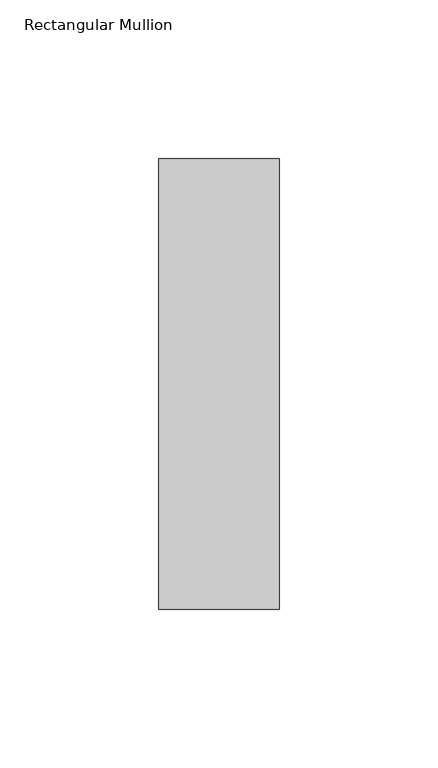
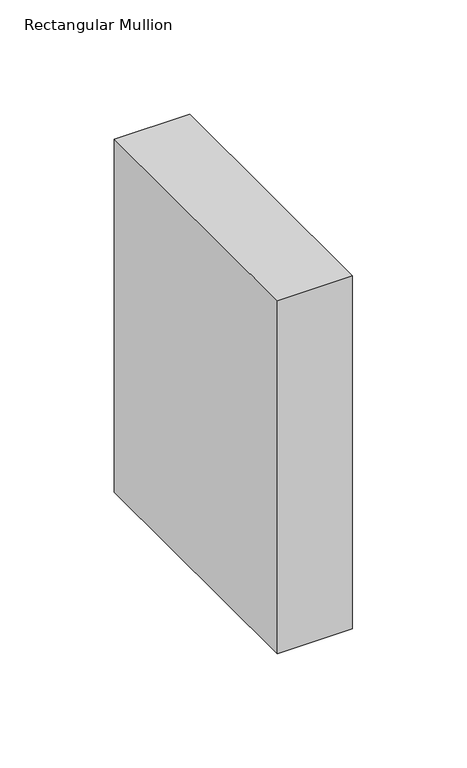
"""IFC4 building model written with IfcOpenShell, lengths in millimetres: member geometry, Rectangular Mullion : NLRS_21_CWM_hsb-regel 38x142_gen_rsf."""

from ifc_helpers import new_model, si_unit, frame, origin, place, context, project, spatial, polyline, outline, extrude, source, transform, mapped, element, save


def rectangular_mullion_db279188(model_context):
    return source(origin(), model_context, "Body", "SweptSolid", [
        extrude(outline(polyline([(-38.0, -71.0), (-38.0, 71.0), (0.0, 71.0), (0.0, -71.0), (-38.0, -71.0)])), frame((0.0, 0.0, -187.9999997), z_axis=(0.0, 0.0, 1.0), x_axis=(1.0, 0.0, 0.0)), (0.0, 0.0, 1.0), 187.9999997),
    ])


if __name__ == "__main__":
    model = new_model("IFC4")
    model_context = context("Model", 3, world=origin())
    ifc_project = project(units=[si_unit("LENGTHUNIT", "METRE", prefix="MILLI")], contexts=[model_context])
    site = spatial("IfcSite", under=ifc_project)
    building = spatial("IfcBuilding", under=site)
    placement = place(None, origin())
    rectangular_mullion_shape = rectangular_mullion_db279188(model_context)
    element("IfcMember", 1, ObjectType="Rectangular Mullion : NLRS_21_CWM_hsb-regel 38x142_gen_rsf", at=placement, inside=building, context=model_context, shape_type="MappedRepresentation", body=[
        mapped(rectangular_mullion_shape, transform((0.0, 0.0, 0.0), x_axis=(1.0, 0.0, 0.0), y_axis=(0.0, 1.0, 0.0), z_axis=(0.0, 0.0, 1.0))),
    ])
    save(model, "model.ifc")

# Revit data of these elements
# Type "Rectangular Mullion : NLRS_21_CWM_hsb-regel 38x142_gen_rsf"
#   Export Type to IFC As = "IfcWall"
#   Type IfcGUID = "07M7mRoiH1CR8m_RSKIwpF"
#   Assembly Code = "21.10"
#   built-in parameter 1007322 = 0.465879 (stored number, unit not read)
#   built-in parameter 1007321 = 0.062336 (stored number, unit not read)
#   built-in parameter 1007320 = 0.062336 (stored number, unit not read)
# Element 1 (IfcMember, "Rectangular Mullion : NLRS_21_CWM_hsb-regel 38x142_gen_rsf")
#   Materials on its faces: "NLRS_i2_hout naaldhout vuren_gen_rsf"
# Materials
#   "NLRS_i2_hout naaldhout vuren_gen_rsf": class "I - Hout", colour RGB 234 199 147, transparency 0, Keynote = "i2", Manufacturer = "Revit Standards Foundation", URL = "www.revitstandards.org", Description = "hout vuren", Cost = 0
